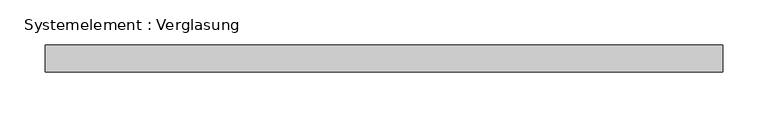
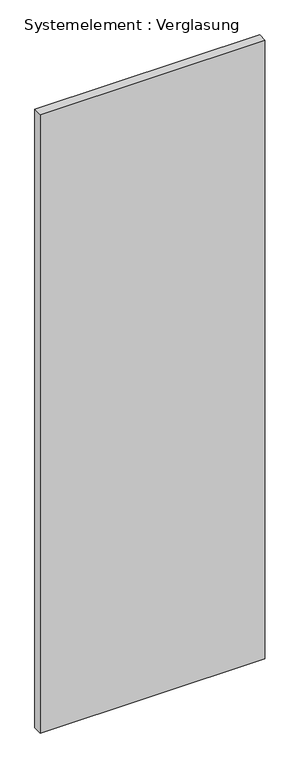
"""IFC4 building model written with IfcOpenShell, lengths in millimetres: plate geometry, Systemelement : Verglasung."""

from ifc_helpers import new_model, si_unit, origin, origin_with_axes, place, context, project, spatial, polyline, outline, extrude, source, transform, mapped, element, save


def systemelement_verglasung_613a1371(model_context):
    return source(origin(), model_context, "Body", "SweptSolid", [
        extrude(outline(polyline([(376.4731315, -15.0), (-376.4731315, -15.0), (-376.4731315, 15.0), (376.4731315, 15.0), (376.4731315, -15.0)])), origin_with_axes(), (0.0, 0.0, 1.0), 2190.0),
    ])


if __name__ == "__main__":
    model = new_model("IFC4")
    model_context = context("Model", 3, world=origin())
    ifc_project = project(units=[si_unit("LENGTHUNIT", "METRE", prefix="MILLI")], contexts=[model_context])
    site = spatial("IfcSite", under=ifc_project)
    building = spatial("IfcBuilding", under=site)
    placement = place(None, origin())
    systemelement_verglasung_shape = systemelement_verglasung_613a1371(model_context)
    element("IfcPlate", 1, ObjectType="Systemelement : Verglasung", at=placement, inside=building, context=model_context, shape_type="MappedRepresentation", body=[
        mapped(systemelement_verglasung_shape, transform((0.0, 0.0, 0.0), x_axis=(1.0, 0.0, 0.0), y_axis=(0.0, 1.0, 0.0), z_axis=(0.0, 0.0, 1.0))),
    ])
    save(model, "model.ifc")

# Revit data of these elements
# Type "Systemelement : Verglasung"
#   Construction Type Id = "GSP4R"
#   Analytic Construction = "1/8 Zoll Pilkington-Verglasung einfach"
#   Visual Light Transmittance = 0.9
#   Solar Heat Gain Coefficient = 0.86
#   Heat Transfer Coefficient (U) = 6.7069 W/(m²·K)
# Element 1 (IfcPlate, "Systemelement : Verglasung")
#   Materials on its faces: "Glas"
# Materials
#   "Glas": class "Glas", colour RGB 0 0 255, transparency 0.75, Comments = "Render-Darstellung nicht aktualisiert ", Cost = 0
